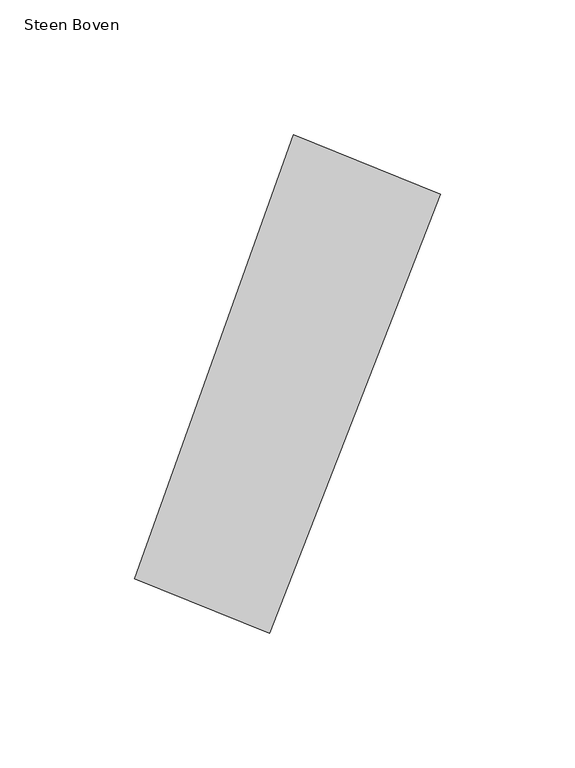
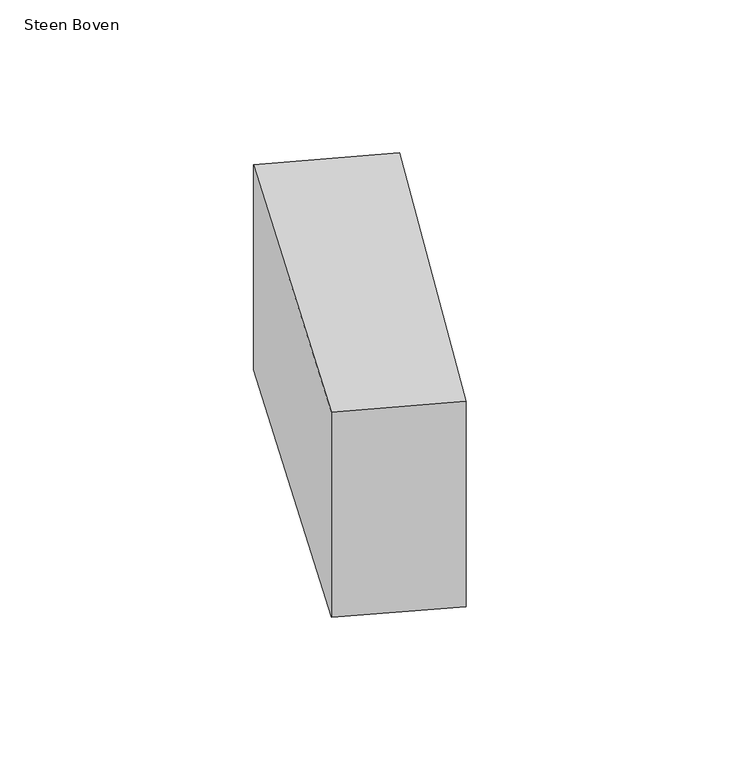
"""IFC4 building model written with IfcOpenShell, lengths in millimetres: proxy geometry, 00_GMA_steen_versie_4 : Steen Boven."""

from ifc_helpers import new_model, si_unit, origin, origin_with_axes, place, context, project, spatial, polyline, outline, extrude, source, transform, mapped, element, save


def steen_boven_f1e39715(model_context):
    return source(origin(), model_context, "Body", "SweptSolid", [
        extrude(outline(polyline([(133.6191629, 154.3357446), (70.0376369, -8.7240178), (19.8735532, 11.6343183), (78.9829907, 176.5127802), (133.6191629, 154.3357446)])), origin_with_axes(), (0.0, 0.0, 1.0), 100.0),
    ])


if __name__ == "__main__":
    model = new_model("IFC4")
    model_context = context("Model", 3, world=origin())
    ifc_project = project(units=[si_unit("LENGTHUNIT", "METRE", prefix="MILLI")], contexts=[model_context])
    site = spatial("IfcSite", under=ifc_project)
    building = spatial("IfcBuilding", under=site)
    placement = place(None, origin())
    steen_boven_shape = steen_boven_f1e39715(model_context)
    element("IfcBuildingElementProxy", 1, Name="00_GMA_steen_versie_4 : Steen Boven", ObjectType="00_GMA_steen_versie_4 : Steen Boven", at=placement, inside=building, context=model_context, shape_type="MappedRepresentation", body=[
        mapped(steen_boven_shape, transform((0.0, 0.0, 0.0), x_axis=(1.0, 0.0, 0.0), y_axis=(0.0, 1.0, 0.0), z_axis=(0.0, 0.0, 1.0))),
    ])
    save(model, "model.ifc")

# Revit data of these elements
# Type "00_GMA_steen_versie_4 : Steen Boven"
#   StootVoegHalfBoven [instance default] = 5 mm
#   StootVoegHalf [instance default] = 5 mm
#   StootVoegBreedteOnder = 10 mm
#   StootVoegBreedteBoven = 10 mm
#   Steendikte = 100 mm
#   LintVoegOnderHalf = 5 mm
#   LintVoegOnder = 10 mm
#   LintVoegBovenHalf = 0 mm
#   LintVoegBoven = 0 mm
#   materiaal = none
#   MateriaalVoeg = none
#   Default Elevation = 0
